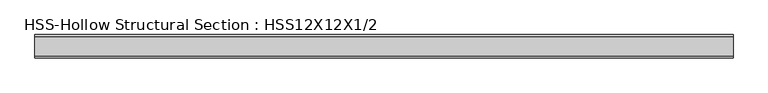
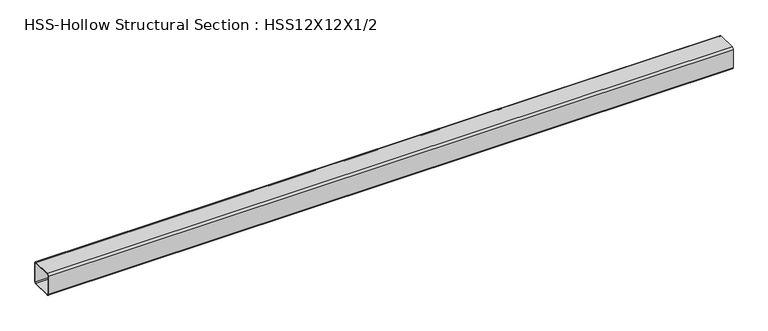
"""IFC4 building model written with IfcOpenShell, lengths in millimetres: beam geometry, HSS-Hollow Structural Section : HSS12X12X1/2."""

from ifc_helpers import new_model, si_unit, point, frame, frame_2d, origin, place, context, project, spatial, polyline, circle_curve, trimmed, segment, composite_curve, outline, extrude, source, transform, mapped, element, save


def hss_hollow_structural_section_hss12x12x1_2_c205e00b(model_context):
    return source(origin(), model_context, "Body", "SweptSolid", [
        extrude(outline(composite_curve([segment(polyline([(152.4, 128.778), (152.4, -128.778)]), True, "CONTINUOUS"), segment(trimmed(circle_curve(frame_2d((128.778, -128.778)), 23.622), [point((152.4, -128.778))], [point((128.778, -152.4))], False, "CARTESIAN"), True, "CONTINUOUS"), segment(polyline([(128.778, -152.4), (-128.778, -152.4)]), True, "CONTINUOUS"), segment(trimmed(circle_curve(frame_2d((-128.778, -128.778)), 23.622), [point((-128.778, -152.4))], [point((-152.4, -128.778))], False, "CARTESIAN"), True, "CONTINUOUS"), segment(polyline([(-152.4, -128.778), (-152.4, 128.778)]), True, "CONTINUOUS"), segment(trimmed(circle_curve(frame_2d((-128.778, 128.778)), 23.622), [point((-152.4, 128.778))], [point((-128.778, 152.4))], False, "CARTESIAN"), True, "CONTINUOUS"), segment(polyline([(-128.778, 152.4), (128.778, 152.4)]), True, "CONTINUOUS"), segment(trimmed(circle_curve(frame_2d((128.778, 128.778)), 23.622), [point((128.778, 152.4))], [point((152.4, 128.778))], False, "CARTESIAN"), True, "CONTINUOUS")], self_intersect=False), holes=[composite_curve([segment(trimmed(circle_curve(frame_2d((-128.778, 128.778)), 11.811), [point((-128.778, 140.589))], [point((-140.589, 128.778))], True, "CARTESIAN"), True, "CONTINUOUS"), segment(polyline([(-140.589, 128.778), (-140.589, -128.778)]), True, "CONTINUOUS"), segment(trimmed(circle_curve(frame_2d((-128.778, -128.778)), 11.811), [point((-140.589, -128.778))], [point((-128.778, -140.589))], True, "CARTESIAN"), True, "CONTINUOUS"), segment(polyline([(-128.778, -140.589), (128.778, -140.589)]), True, "CONTINUOUS"), segment(trimmed(circle_curve(frame_2d((128.778, -128.778)), 11.811), [point((128.778, -140.589))], [point((140.589, -128.778))], True, "CARTESIAN"), True, "CONTINUOUS"), segment(polyline([(140.589, -128.778), (140.589, 128.778)]), True, "CONTINUOUS"), segment(trimmed(circle_curve(frame_2d((128.778, 128.778)), 11.811), [point((140.589, 128.778))], [point((128.778, 140.589))], True, "CARTESIAN"), True, "CONTINUOUS"), segment(polyline([(128.778, 140.589), (-128.778, 140.589)]), True, "CONTINUOUS")], self_intersect=False)]), frame((-4648.2, 0.0, 0.0), z_axis=(1.0, 0.0, 0.0), x_axis=(0.0, 1.0, 0.0)), (0.0, 0.0, 1.0), 9144.0),
    ])


if __name__ == "__main__":
    model = new_model("IFC4")
    model_context = context("Model", 3, world=origin())
    ifc_project = project(units=[si_unit("LENGTHUNIT", "METRE", prefix="MILLI")], contexts=[model_context])
    site = spatial("IfcSite", under=ifc_project)
    building = spatial("IfcBuilding", under=site)
    placement = place(None, origin())
    hss_hollow_structural_section_hss12x12x1_2_shape = hss_hollow_structural_section_hss12x12x1_2_c205e00b(model_context)
    element("IfcBeam", 1, ObjectType="HSS-Hollow Structural Section : HSS12X12X1/2", at=placement, inside=building, context=model_context, shape_type="MappedRepresentation", body=[
        mapped(hss_hollow_structural_section_hss12x12x1_2_shape, transform((0.0, 0.0, 0.0), x_axis=(1.0, 0.0, 0.0), y_axis=(0.0, 1.0, 0.0), z_axis=(0.0, 0.0, 1.0))),
    ])
    save(model, "model.ifc")

# Revit data of these elements
# Type "HSS-Hollow Structural Section : HSS12X12X1/2"
#   Assembly Code = "B10"
#   Shape = "Square"
#   W = 75.9
#   Ht = 304.8 mm
#   Length [instance default] = 1524 mm
#   b = 304.8 mm
#   kr = 23.622 mm
#   t = 11.811 mm
#   A = 0.0134838 m²
#   Structural Material [instance default] = Steel ASTM A500, Grade B, Rectangular and Square
# Element 1 (IfcBeam, "HSS-Hollow Structural Section : HSS12X12X1/2")
#   Structural Material = Aluminum 7175 T73 0 Hot Formed
#   Materials on its faces: "Aluminum 7175 T73 0 Hot Formed"
# Materials
#   "Steel ASTM A500, Grade B, Rectangular and Square": class "Metal", colour RGB 199 199 199, transparency 0, Description = "Carbon steel", Cost = 0
#   "Aluminum 7175 T73 0 Hot Formed": class "Metal", colour RGB 120 120 120, transparency 0, Description = "Physical material.", Cost = 0
